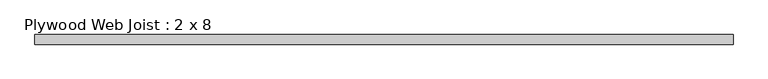
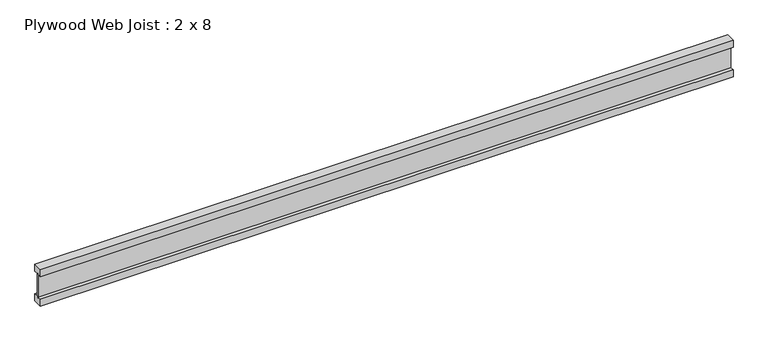
"""IFC4 building model written with IfcOpenShell, lengths in millimetres: beam geometry, Plywood Web Joist : 2 x 8."""

import ifcopenshell
import ifcopenshell.guid

model = None  # the IFC model being written
_history = None  # IfcOwnerHistory: only IFC2X3 demands one
_inside = {}  # id of a spatial element -> (the spatial element, [elements in it])
_under = {}  # id of a project, library or spatial element -> (it, [spatial elements below it])
_declared = {}  # id of a project -> (the project, [libraries it declares])
_typed = {}  # id of a type object -> (the type object, [elements of that type])
_made_of = {}  # id of a material, layer set ... -> (it, [elements and type objects made of it])


def new_model(schema):
    """Start an empty IFC model of exactly this schema.

    Asked for "IFC4X3", IfcOpenShell would pick the latest addendum, in which some entities
    have other attributes; the version numbers below select the first issue.
    IFC2X3 requires an IfcOwnerHistory on every rooted entity: one is made here for all.
    """
    global model, _history
    if schema == "IFC4X3":
        model = ifcopenshell.file(schema_version=(4, 3, 0, 0))
    else:
        model = ifcopenshell.file(schema=schema)
    _inside.clear()
    _under.clear()
    _declared.clear()
    _typed.clear()
    _made_of.clear()
    _history = None
    if model.schema == "IFC2X3":
        org = make("IfcOrganization", Name="unknown")
        user = make(
            "IfcPersonAndOrganization",
            ThePerson=make("IfcPerson", FamilyName="unknown"),
            TheOrganization=org,
        )
        app = make(
            "IfcApplication",
            ApplicationDeveloper=org,
            Version="unknown",
            ApplicationFullName="unknown",
            ApplicationIdentifier="unknown",
        )
        _history = make(
            "IfcOwnerHistory",
            OwningUser=user,
            OwningApplication=app,
            ChangeAction="ADDED",
            CreationDate=0,
        )
    return model


def make(cls, **values):
    """One entity of the class cls with the attributes given. An attribute that is None is left unset."""
    return model.create_entity(
        cls, **{name: value for name, value in values.items() if value is not None}
    )


def rooted(cls, **values):
    """An entity with a GlobalId (a new one), such as an element, a storey or a relation."""
    return make(cls, GlobalId=ifcopenshell.guid.new(), OwnerHistory=_history, **values)


def si_unit(unit_type, name, prefix=None):
    """IfcSIUnit, for example si_unit("LENGTHUNIT", "METRE", prefix="MILLI")."""
    return make("IfcSIUnit", UnitType=unit_type, Prefix=prefix, Name=name)


def assignment(units):
    """IfcUnitAssignment: the units of a project."""
    return None if units is None else make("IfcUnitAssignment", Units=units)


def point(xyz):
    """IfcCartesianPoint."""
    return None if xyz is None else make("IfcCartesianPoint", Coordinates=xyz)


def direction(xyz):
    """IfcDirection."""
    return None if xyz is None else make("IfcDirection", DirectionRatios=xyz)


def frame(location, z_axis=None, x_axis=None):
    """IfcAxis2Placement3D, a coordinate frame: its origin and axes. An axis left out is left unset."""
    return make(
        "IfcAxis2Placement3D",
        Location=point(location),
        Axis=direction(z_axis),
        RefDirection=direction(x_axis),
    )


def origin():
    """The frame at (0, 0, 0) with its axes left unset."""
    return frame((0.0, 0.0, 0.0))


def place(relative_to, where):
    """IfcLocalPlacement: puts the frame where relative to a parent placement (None: the world)."""
    return make(
        "IfcLocalPlacement", PlacementRelTo=relative_to, RelativePlacement=where
    )


def context(
    kind, dimensions, precision=None, world=None, true_north=None, identifier=None
):
    """IfcGeometricRepresentationContext, for example the 3D "Model" context."""
    return make(
        "IfcGeometricRepresentationContext",
        ContextIdentifier=identifier,
        ContextType=kind,
        CoordinateSpaceDimension=dimensions,
        Precision=precision,
        WorldCoordinateSystem=world,
        TrueNorth=true_north,
    )


def project(units=None, contexts=None):
    """IfcProject with its units and contexts."""
    return rooted(
        "IfcProject",
        Name="project",
        RepresentationContexts=contexts,
        UnitsInContext=assignment(units),
    )


def spatial(cls, under=None, at=None, **own):
    """A site, building, storey or space (cls), placed at a placement, below another one or the project."""
    s = rooted(cls, ObjectPlacement=at, **own)
    if under is not None:
        _under.setdefault(under.id(), (under, []))[1].append(s)
    return s


def polyline(points):
    """IfcPolyline through the points."""
    return make("IfcPolyline", Points=[point(p) for p in points])


def outline(outer, holes=None, kind="AREA"):
    """IfcArbitraryClosedProfileDef: a profile drawn as a closed curve; with holes, ...WithVoids."""
    if holes is None:
        return make("IfcArbitraryClosedProfileDef", ProfileType=kind, OuterCurve=outer)
    return make(
        "IfcArbitraryProfileDefWithVoids",
        ProfileType=kind,
        OuterCurve=outer,
        InnerCurves=holes,
    )


def extrude(swept, where, along, depth):
    """IfcExtrudedAreaSolid: the profile swept, set in the frame where, extruded along a direction by depth."""
    return make(
        "IfcExtrudedAreaSolid",
        SweptArea=swept,
        Position=where,
        ExtrudedDirection=direction(along),
        Depth=depth,
    )


def shape(context_of_items, identifier, shape_type, items):
    """IfcShapeRepresentation: the items that make up one representation, for example the "Body"."""
    return make(
        "IfcShapeRepresentation",
        ContextOfItems=context_of_items,
        RepresentationIdentifier=identifier,
        RepresentationType=shape_type,
        Items=items,
    )


def source(mapping_origin, context_of_items, identifier, shape_type, items):
    """IfcRepresentationMap: a shape defined once, which mapped items show again and again."""
    return make(
        "IfcRepresentationMap",
        MappingOrigin=mapping_origin,
        MappedRepresentation=shape(context_of_items, identifier, shape_type, items),
    )


def transform(
    local_origin,
    x_axis=None,
    y_axis=None,
    z_axis=None,
    scale=None,
    scale2=None,
    scale3=None,
    uniform=True,
):
    """IfcCartesianTransformationOperator3D, or its non-uniform kind. x_axis, y_axis, z_axis: its Axis1, 2, 3."""
    if uniform:
        return make(
            "IfcCartesianTransformationOperator3D",
            Axis1=direction(x_axis),
            Axis2=direction(y_axis),
            LocalOrigin=point(local_origin),
            Scale=scale,
            Axis3=direction(z_axis),
        )
    return make(
        "IfcCartesianTransformationOperator3DnonUniform",
        Axis1=direction(x_axis),
        Axis2=direction(y_axis),
        LocalOrigin=point(local_origin),
        Scale=scale,
        Axis3=direction(z_axis),
        Scale2=scale2,
        Scale3=scale3,
    )


def mapped(mapping_source, mapping_target):
    """IfcMappedItem: shows the shape of a source again, moved by a transform."""
    return make(
        "IfcMappedItem", MappingSource=mapping_source, MappingTarget=mapping_target
    )


def made_of(thing, what):
    """Note that an element or type object is made of a material, layer set ...; save() writes the relation."""
    if what is not None:
        _made_of.setdefault(what.id(), (what, []))[1].append(thing)
    return thing


def element(
    cls,
    number,
    at=None,
    inside=None,
    cuts=None,
    type_object=None,
    material=None,
    context=None,
    identifier="Body",
    shape_type=None,
    held_by="IfcProductDefinitionShape",
    body=None,
    shapes=None,
    **own,
):
    """One element of the class cls, such as IfcWall. Its Tag is "e" and its number.

    at: its placement. inside: the storey or other place that contains it. cuts: it is an
    opening in that element (IfcRelVoidsElement). A single representation is given by context,
    identifier, shape_type and body (its items); several are given by shapes. held_by: the class
    of the entity that holds the representations. save() writes the other relations.
    """
    e = rooted(cls, Tag="e%d" % number, ObjectPlacement=at, **own)
    if body is not None:
        shapes = [shape(context, identifier, shape_type, body)]
    if shapes is not None:
        e.Representation = make(held_by, Representations=shapes)
    if inside is not None:
        _inside.setdefault(inside.id(), (inside, []))[1].append(e)
    if cuts is not None:
        rooted(
            "IfcRelVoidsElement", RelatingBuildingElement=cuts, RelatedOpeningElement=e
        )
    if type_object is not None:
        _typed.setdefault(type_object.id(), (type_object, []))[1].append(e)
    return made_of(e, material)


def aggregate(whole, parts):
    """IfcRelAggregates: a whole, such as a stair, and the parts it consists of."""
    return rooted("IfcRelAggregates", RelatingObject=whole, RelatedObjects=parts)


def save(model, path):
    """Write the relations noted so far, then the file.

    IfcRelAggregates (storeys below a building ...), IfcRelContainedInSpatialStructure (elements
    in a storey), IfcRelDefinesByType, IfcRelAssociatesMaterial and IfcRelDeclares: one each for
    every whole, place, type object, material and project.
    """
    for whole, parts in _under.values():
        aggregate(whole, parts)
    for where, things in _inside.values():
        rooted(
            "IfcRelContainedInSpatialStructure",
            RelatedElements=things,
            RelatingStructure=where,
        )
    for kind, things in _typed.values():
        rooted("IfcRelDefinesByType", RelatedObjects=things, RelatingType=kind)
    for what, things in _made_of.values():
        rooted("IfcRelAssociatesMaterial", RelatedObjects=things, RelatingMaterial=what)
    for by, libraries in _declared.values():
        rooted("IfcRelDeclares", RelatingContext=by, RelatedDefinitions=libraries)
    model.write(path)


def plywood_web_joist_2_x_8_093a3c26(model_context):
    return source(origin(), model_context, "Body", "SweptSolid", [
        extrude(outline(polyline([(-25.4, 101.6), (25.4, 101.6), (25.4, 63.5), (4.7625, 63.5), (4.7625, 69.85), (-4.7625, 69.85), (-4.7625, 63.5), (-25.4, 63.5), (-25.4, 101.6)])), frame((-1835.15, 0.0, 0.0), z_axis=(1.0, 0.0, 0.0), x_axis=(0.0, 1.0, 0.0)), (0.0, 0.0, 1.0), 3670.3),
        extrude(outline(polyline([(25.4, -63.5), (25.4, -101.6), (-25.4, -101.6), (-25.4, -63.5), (-4.7625, -63.5), (-4.7625, -69.1160374), (4.7625, -69.1160374), (4.7625, -63.5), (25.4, -63.5)])), frame((-1835.15, 0.0, 0.0), z_axis=(1.0, 0.0, 0.0), x_axis=(0.0, 1.0, 0.0)), (0.0, 0.0, 1.0), 3670.3),
        extrude(outline(polyline([(1835.15, 4.7625), (1835.15, -4.7625), (-1835.15, -4.7625), (-1835.15, 4.7625), (1835.15, 4.7625)])), frame((0.0, 0.0, -69.1160374), z_axis=(0.0, 0.0, 1.0), x_axis=(1.0, 0.0, 0.0)), (0.0, 0.0, 1.0), 138.9660374),
    ])


if __name__ == "__main__":
    model = new_model("IFC4")
    model_context = context("Model", 3, world=origin())
    ifc_project = project(units=[si_unit("LENGTHUNIT", "METRE", prefix="MILLI")], contexts=[model_context])
    site = spatial("IfcSite", under=ifc_project)
    building = spatial("IfcBuilding", under=site)
    placement = place(None, origin())
    plywood_web_joist_2_x_8_shape = plywood_web_joist_2_x_8_093a3c26(model_context)
    element("IfcBeam", 1, ObjectType="Plywood Web Joist : 2 x 8", at=placement, inside=building, context=model_context, shape_type="MappedRepresentation", body=[
        mapped(plywood_web_joist_2_x_8_shape, transform((0.0, 0.0, 0.0), x_axis=(1.0, 0.0, 0.0), y_axis=(0.0, 1.0, 0.0), z_axis=(0.0, 0.0, 1.0))),
    ])
    save(model, "model.ifc")

# Revit data of these elements
# Project information
#   Project Issue Date = "Issue Date"
#   Project Status = "Project Status"
#   Client Name = "Owner"
#   Project Address = "Enter address here"
#   Project Name = "Project Name"
#   Project Number = "Project Number"
# Type "Plywood Web Joist : 2 x 8"
#   Assembly Code = "B10"
#   Length [instance default] = 5' - 0"
#   b = 0' - 2"
#   d = 0' - 8"
#   Structural Material [instance default] = Softwood, Lumber
# Element 1 (IfcBeam, "Plywood Web Joist : 2 x 8")
#   Materials on its faces: "Softwood, Lumber"
# Materials
#   "Softwood, Lumber": class "Wood", colour RGB 144 113 62, transparency 0, Description = "Pinus Echinata", Cost = 0
